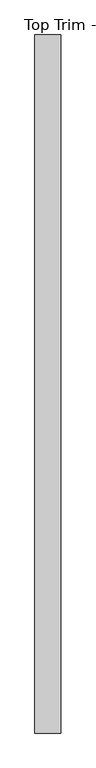
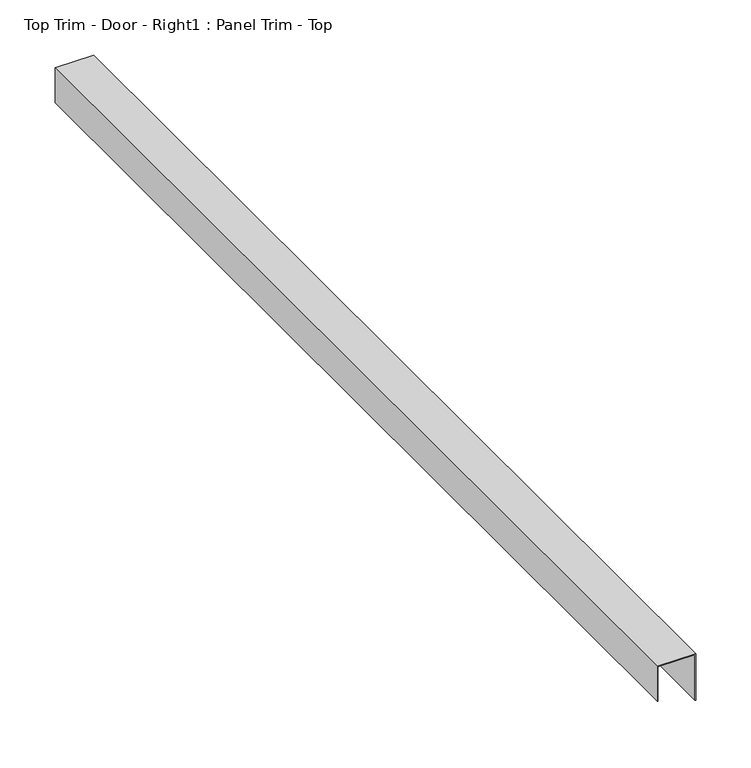
"""IFC4 building model written with IfcOpenShell, lengths in millimetres: proxy geometry, Top Trim - Door - Right1 : Panel Trim - Top."""

from ifc_helpers import new_model, si_unit, frame, origin, place, context, project, spatial, polyline, outline, extrude, source, transform, mapped, element, save


def top_trim_door_right1_panel_trim_top_e01be231(model_context):
    return source(origin(), model_context, "Body", "SweptSolid", [
        extrude(outline(polyline([(2438.4, 587327.0060739), (2438.4, 587365.8934739), (2387.6, 587365.8934739), (2387.6, 587366.6808739), (2439.19375, 587366.6808739), (2439.19375, 587326.2186739), (2400.3, 587326.2186739), (2400.3, 587327.0060739), (2438.4, 587327.0060739)])), frame((0.0, -536301.7038841, 0.0), z_axis=(0.0, 1.0, 0.0), x_axis=(0.0, 0.0, 1.0)), (0.0, 0.0, 1.0), 1093.7875),
    ])


if __name__ == "__main__":
    model = new_model("IFC4")
    model_context = context("Model", 3, world=origin())
    ifc_project = project(units=[si_unit("LENGTHUNIT", "METRE", prefix="MILLI")], contexts=[model_context])
    site = spatial("IfcSite", under=ifc_project)
    building = spatial("IfcBuilding", under=site)
    placement = place(None, origin())
    top_trim_door_right1_panel_trim_top_shape = top_trim_door_right1_panel_trim_top_e01be231(model_context)
    element("IfcBuildingElementProxy", 1, Name="Top Trim - Door - Right1 : Panel Trim - Top", ObjectType="Top Trim - Door - Right1 : Panel Trim - Top", at=placement, inside=building, context=model_context, shape_type="MappedRepresentation", body=[
        mapped(top_trim_door_right1_panel_trim_top_shape, transform((0.0, 0.0, 0.0), x_axis=(1.0, 0.0, 0.0), y_axis=(0.0, 1.0, 0.0), z_axis=(0.0, 0.0, 1.0))),
    ])
    save(model, "model.ifc")

# Revit data of these elements
# Element 1 (IfcBuildingElementProxy, "Top Trim - Door - Right1 : Panel Trim - Top")
#   Materials on its faces: "EDGE TRIM BY MTL PANEL MFR."
# Materials
#   "EDGE TRIM BY MTL PANEL MFR.": class "Generic", colour RGB 239 242 240, transparency 0, Cost = 0
